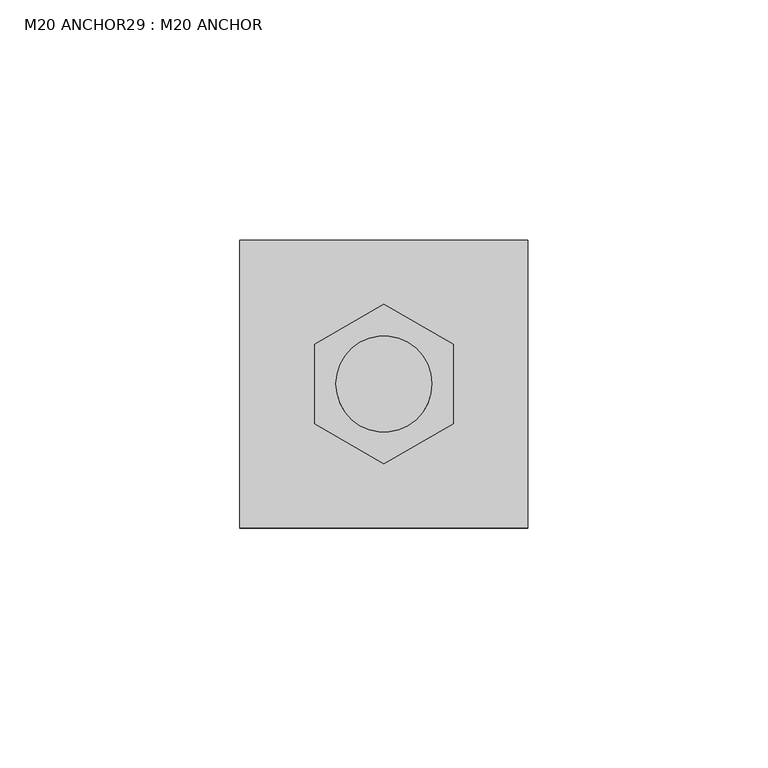
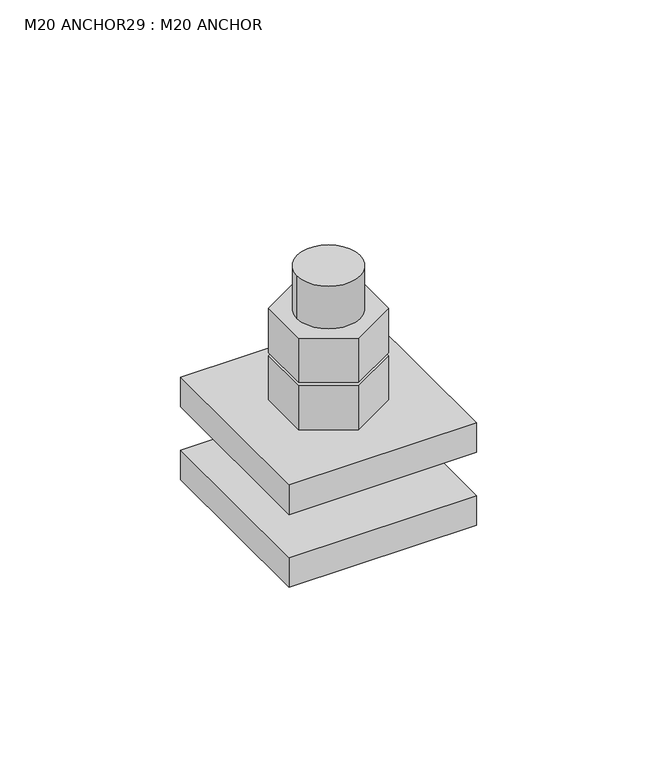
"""IFC4 building model written with IfcOpenShell, lengths in millimetres: fastener geometry, M20 ANCHOR29 : M20 ANCHOR."""

from ifc_helpers import new_model, si_unit, point, frame, frame_2d, origin, place, context, project, spatial, polyline, circle_curve, trimmed, segment, composite_curve, outline, extrude, source, transform, mapped, element, save


def m20_anchor29_m20_anchor_617c0da3(model_context):
    return source(origin(), model_context, "Body", "SweptSolid", [
        extrude(outline(polyline([(-30764.8864916, -7426.8093347), (-30779.2946106, -7435.1278661), (-30793.7027297, -7426.8093347), (-30793.7027297, -7410.1722719), (-30779.2946106, -7401.8537405), (-30764.8864916, -7410.1722719), (-30764.8864916, -7426.8093347)]), holes=[composite_curve([segment(trimmed(circle_curve(frame_2d((-30779.2946106, -7418.4908033)), 10.0), [point((-30789.2946106, -7418.4908033))], [point((-30769.2946106, -7418.4908033))], True, "CARTESIAN"), True, "CONTINUOUS"), segment(trimmed(circle_curve(frame_2d((-30779.2946106, -7418.4908033)), 10.0), [point((-30769.2946106, -7418.4908033))], [point((-30789.2946106, -7418.4908033))], True, "CARTESIAN"), True, "CONTINUOUS")], self_intersect=False)]), frame((0.0, 0.0, 240.605), z_axis=(0.0, 0.0, 1.0), x_axis=(1.0, 0.0, 0.0)), (0.0, 0.0, 1.0), 15.0),
        extrude(outline(polyline([(-30764.8864916, -7426.8093347), (-30779.2946106, -7435.1278661), (-30793.7027297, -7426.8093347), (-30793.7027297, -7410.1722719), (-30779.2946106, -7401.8537405), (-30764.8864916, -7410.1722719), (-30764.8864916, -7426.8093347)]), holes=[composite_curve([segment(trimmed(circle_curve(frame_2d((-30779.2946106, -7418.4908033)), 10.0), [point((-30789.2946106, -7418.4908033))], [point((-30769.2946106, -7418.4908033))], True, "CARTESIAN"), True, "CONTINUOUS"), segment(trimmed(circle_curve(frame_2d((-30779.2946106, -7418.4908033)), 10.0), [point((-30769.2946106, -7418.4908033))], [point((-30789.2946106, -7418.4908033))], True, "CARTESIAN"), True, "CONTINUOUS")], self_intersect=False)]), frame((0.0, 0.0, 224.605), z_axis=(0.0, 0.0, 1.0), x_axis=(1.0, 0.0, 0.0)), (0.0, 0.0, 1.0), 15.0),
        extrude(outline(composite_curve([segment(trimmed(circle_curve(frame_2d((-30779.2946106, -7418.4908033)), 10.0), [point((-30789.2946106, -7418.4908033))], [point((-30769.2946106, -7418.4908033))], False, "CARTESIAN"), True, "CONTINUOUS"), segment(trimmed(circle_curve(frame_2d((-30779.2946106, -7418.4908033)), 10.0), [point((-30769.2946106, -7418.4908033))], [point((-30789.2946106, -7418.4908033))], False, "CARTESIAN"), True, "CONTINUOUS")], self_intersect=False)), frame((0.0, 0.0, 190.0), z_axis=(0.0, 0.0, 1.0), x_axis=(1.0, 0.0, 0.0)), (0.0, 0.0, 1.0), 80.0),
        extrude(outline(polyline([(-30749.2946106, -7448.4908033), (-30809.2946106, -7448.4908033), (-30809.2946106, -7388.4908033), (-30749.2946106, -7388.4908033), (-30749.2946106, -7448.4908033)]), holes=[composite_curve([segment(trimmed(circle_curve(frame_2d((-30779.2946106, -7418.4908033)), 11.0), [point((-30790.2946106, -7418.4908033))], [point((-30768.2946106, -7418.4908033))], True, "CARTESIAN"), True, "CONTINUOUS"), segment(trimmed(circle_curve(frame_2d((-30779.2946106, -7418.4908033)), 11.0), [point((-30768.2946106, -7418.4908033))], [point((-30790.2946106, -7418.4908033))], True, "CARTESIAN"), True, "CONTINUOUS")], self_intersect=False)]), frame((0.0, 0.0, 190.0), z_axis=(0.0, 0.0, 1.0), x_axis=(1.0, 0.0, 0.0)), (0.0, 0.0, 1.0), 10.0),
        extrude(outline(polyline([(-30749.2946106, -7448.4908033), (-30809.2946106, -7448.4908033), (-30809.2946106, -7388.4908033), (-30749.2946106, -7388.4908033), (-30749.2946106, -7448.4908033)]), holes=[composite_curve([segment(trimmed(circle_curve(frame_2d((-30779.2946106, -7418.4908033)), 11.0), [point((-30790.2946106, -7418.4908033))], [point((-30768.2946106, -7418.4908033))], True, "CARTESIAN"), True, "CONTINUOUS"), segment(trimmed(circle_curve(frame_2d((-30779.2946106, -7418.4908033)), 11.0), [point((-30768.2946106, -7418.4908033))], [point((-30790.2946106, -7418.4908033))], True, "CARTESIAN"), True, "CONTINUOUS")], self_intersect=False)]), frame((0.0, 0.0, 214.605), z_axis=(0.0, 0.0, 1.0), x_axis=(1.0, 0.0, 0.0)), (0.0, 0.0, 1.0), 10.0),
    ])


if __name__ == "__main__":
    model = new_model("IFC4")
    model_context = context("Model", 3, world=origin())
    ifc_project = project(units=[si_unit("LENGTHUNIT", "METRE", prefix="MILLI")], contexts=[model_context])
    site = spatial("IfcSite", under=ifc_project)
    building = spatial("IfcBuilding", under=site)
    placement = place(None, origin())
    m20_anchor29_m20_anchor_shape = m20_anchor29_m20_anchor_617c0da3(model_context)
    element("IfcFastener", 1, ObjectType="M20 ANCHOR29 : M20 ANCHOR", at=placement, inside=building, context=model_context, shape_type="MappedRepresentation", body=[
        mapped(m20_anchor29_m20_anchor_shape, transform((0.0, 0.0, 0.0), x_axis=(1.0, 0.0, 0.0), y_axis=(0.0, 1.0, 0.0), z_axis=(0.0, 0.0, 1.0))),
    ])
    save(model, "model.ifc")
